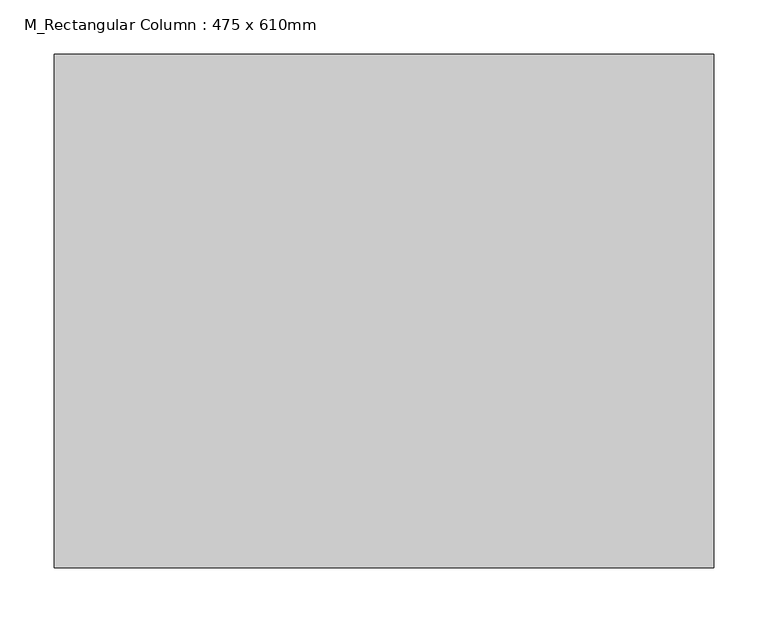
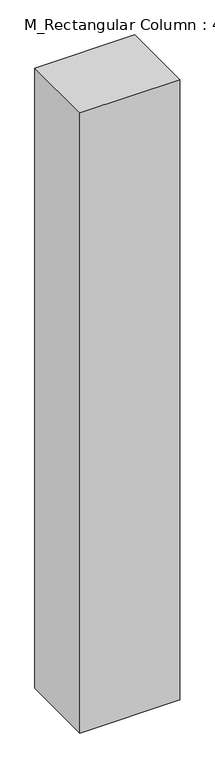
"""IFC4 building model written with IfcOpenShell, lengths in millimetres: column geometry, M_Rectangular Column : 475 x 610mm."""

import ifcopenshell
import ifcopenshell.guid

model = None  # the IFC model being written
_history = None  # IfcOwnerHistory: only IFC2X3 demands one
_inside = {}  # id of a spatial element -> (the spatial element, [elements in it])
_under = {}  # id of a project, library or spatial element -> (it, [spatial elements below it])
_declared = {}  # id of a project -> (the project, [libraries it declares])
_typed = {}  # id of a type object -> (the type object, [elements of that type])
_made_of = {}  # id of a material, layer set ... -> (it, [elements and type objects made of it])


def new_model(schema):
    """Start an empty IFC model of exactly this schema.

    Asked for "IFC4X3", IfcOpenShell would pick the latest addendum, in which some entities
    have other attributes; the version numbers below select the first issue.
    IFC2X3 requires an IfcOwnerHistory on every rooted entity: one is made here for all.
    """
    global model, _history
    if schema == "IFC4X3":
        model = ifcopenshell.file(schema_version=(4, 3, 0, 0))
    else:
        model = ifcopenshell.file(schema=schema)
    _inside.clear()
    _under.clear()
    _declared.clear()
    _typed.clear()
    _made_of.clear()
    _history = None
    if model.schema == "IFC2X3":
        org = make("IfcOrganization", Name="unknown")
        user = make(
            "IfcPersonAndOrganization",
            ThePerson=make("IfcPerson", FamilyName="unknown"),
            TheOrganization=org,
        )
        app = make(
            "IfcApplication",
            ApplicationDeveloper=org,
            Version="unknown",
            ApplicationFullName="unknown",
            ApplicationIdentifier="unknown",
        )
        _history = make(
            "IfcOwnerHistory",
            OwningUser=user,
            OwningApplication=app,
            ChangeAction="ADDED",
            CreationDate=0,
        )
    return model


def make(cls, **values):
    """One entity of the class cls with the attributes given. An attribute that is None is left unset."""
    return model.create_entity(
        cls, **{name: value for name, value in values.items() if value is not None}
    )


def rooted(cls, **values):
    """An entity with a GlobalId (a new one), such as an element, a storey or a relation."""
    return make(cls, GlobalId=ifcopenshell.guid.new(), OwnerHistory=_history, **values)


def si_unit(unit_type, name, prefix=None):
    """IfcSIUnit, for example si_unit("LENGTHUNIT", "METRE", prefix="MILLI")."""
    return make("IfcSIUnit", UnitType=unit_type, Prefix=prefix, Name=name)


def assignment(units):
    """IfcUnitAssignment: the units of a project."""
    return None if units is None else make("IfcUnitAssignment", Units=units)


def point(xyz):
    """IfcCartesianPoint."""
    return None if xyz is None else make("IfcCartesianPoint", Coordinates=xyz)


def direction(xyz):
    """IfcDirection."""
    return None if xyz is None else make("IfcDirection", DirectionRatios=xyz)


def frame(location, z_axis=None, x_axis=None):
    """IfcAxis2Placement3D, a coordinate frame: its origin and axes. An axis left out is left unset."""
    return make(
        "IfcAxis2Placement3D",
        Location=point(location),
        Axis=direction(z_axis),
        RefDirection=direction(x_axis),
    )


def origin():
    """The frame at (0, 0, 0) with its axes left unset."""
    return frame((0.0, 0.0, 0.0))


def place(relative_to, where):
    """IfcLocalPlacement: puts the frame where relative to a parent placement (None: the world)."""
    return make(
        "IfcLocalPlacement", PlacementRelTo=relative_to, RelativePlacement=where
    )


def context(
    kind, dimensions, precision=None, world=None, true_north=None, identifier=None
):
    """IfcGeometricRepresentationContext, for example the 3D "Model" context."""
    return make(
        "IfcGeometricRepresentationContext",
        ContextIdentifier=identifier,
        ContextType=kind,
        CoordinateSpaceDimension=dimensions,
        Precision=precision,
        WorldCoordinateSystem=world,
        TrueNorth=true_north,
    )


def project(units=None, contexts=None):
    """IfcProject with its units and contexts."""
    return rooted(
        "IfcProject",
        Name="project",
        RepresentationContexts=contexts,
        UnitsInContext=assignment(units),
    )


def spatial(cls, under=None, at=None, **own):
    """A site, building, storey or space (cls), placed at a placement, below another one or the project."""
    s = rooted(cls, ObjectPlacement=at, **own)
    if under is not None:
        _under.setdefault(under.id(), (under, []))[1].append(s)
    return s


def polyline(points):
    """IfcPolyline through the points."""
    return make("IfcPolyline", Points=[point(p) for p in points])


def outline(outer, holes=None, kind="AREA"):
    """IfcArbitraryClosedProfileDef: a profile drawn as a closed curve; with holes, ...WithVoids."""
    if holes is None:
        return make("IfcArbitraryClosedProfileDef", ProfileType=kind, OuterCurve=outer)
    return make(
        "IfcArbitraryProfileDefWithVoids",
        ProfileType=kind,
        OuterCurve=outer,
        InnerCurves=holes,
    )


def extrude(swept, where, along, depth):
    """IfcExtrudedAreaSolid: the profile swept, set in the frame where, extruded along a direction by depth."""
    return make(
        "IfcExtrudedAreaSolid",
        SweptArea=swept,
        Position=where,
        ExtrudedDirection=direction(along),
        Depth=depth,
    )


def shape(context_of_items, identifier, shape_type, items):
    """IfcShapeRepresentation: the items that make up one representation, for example the "Body"."""
    return make(
        "IfcShapeRepresentation",
        ContextOfItems=context_of_items,
        RepresentationIdentifier=identifier,
        RepresentationType=shape_type,
        Items=items,
    )


def source(mapping_origin, context_of_items, identifier, shape_type, items):
    """IfcRepresentationMap: a shape defined once, which mapped items show again and again."""
    return make(
        "IfcRepresentationMap",
        MappingOrigin=mapping_origin,
        MappedRepresentation=shape(context_of_items, identifier, shape_type, items),
    )


def transform(
    local_origin,
    x_axis=None,
    y_axis=None,
    z_axis=None,
    scale=None,
    scale2=None,
    scale3=None,
    uniform=True,
):
    """IfcCartesianTransformationOperator3D, or its non-uniform kind. x_axis, y_axis, z_axis: its Axis1, 2, 3."""
    if uniform:
        return make(
            "IfcCartesianTransformationOperator3D",
            Axis1=direction(x_axis),
            Axis2=direction(y_axis),
            LocalOrigin=point(local_origin),
            Scale=scale,
            Axis3=direction(z_axis),
        )
    return make(
        "IfcCartesianTransformationOperator3DnonUniform",
        Axis1=direction(x_axis),
        Axis2=direction(y_axis),
        LocalOrigin=point(local_origin),
        Scale=scale,
        Axis3=direction(z_axis),
        Scale2=scale2,
        Scale3=scale3,
    )


def mapped(mapping_source, mapping_target):
    """IfcMappedItem: shows the shape of a source again, moved by a transform."""
    return make(
        "IfcMappedItem", MappingSource=mapping_source, MappingTarget=mapping_target
    )


def made_of(thing, what):
    """Note that an element or type object is made of a material, layer set ...; save() writes the relation."""
    if what is not None:
        _made_of.setdefault(what.id(), (what, []))[1].append(thing)
    return thing


def element(
    cls,
    number,
    at=None,
    inside=None,
    cuts=None,
    type_object=None,
    material=None,
    context=None,
    identifier="Body",
    shape_type=None,
    held_by="IfcProductDefinitionShape",
    body=None,
    shapes=None,
    **own,
):
    """One element of the class cls, such as IfcWall. Its Tag is "e" and its number.

    at: its placement. inside: the storey or other place that contains it. cuts: it is an
    opening in that element (IfcRelVoidsElement). A single representation is given by context,
    identifier, shape_type and body (its items); several are given by shapes. held_by: the class
    of the entity that holds the representations. save() writes the other relations.
    """
    e = rooted(cls, Tag="e%d" % number, ObjectPlacement=at, **own)
    if body is not None:
        shapes = [shape(context, identifier, shape_type, body)]
    if shapes is not None:
        e.Representation = make(held_by, Representations=shapes)
    if inside is not None:
        _inside.setdefault(inside.id(), (inside, []))[1].append(e)
    if cuts is not None:
        rooted(
            "IfcRelVoidsElement", RelatingBuildingElement=cuts, RelatedOpeningElement=e
        )
    if type_object is not None:
        _typed.setdefault(type_object.id(), (type_object, []))[1].append(e)
    return made_of(e, material)


def aggregate(whole, parts):
    """IfcRelAggregates: a whole, such as a stair, and the parts it consists of."""
    return rooted("IfcRelAggregates", RelatingObject=whole, RelatedObjects=parts)


def save(model, path):
    """Write the relations noted so far, then the file.

    IfcRelAggregates (storeys below a building ...), IfcRelContainedInSpatialStructure (elements
    in a storey), IfcRelDefinesByType, IfcRelAssociatesMaterial and IfcRelDeclares: one each for
    every whole, place, type object, material and project.
    """
    for whole, parts in _under.values():
        aggregate(whole, parts)
    for where, things in _inside.values():
        rooted(
            "IfcRelContainedInSpatialStructure",
            RelatedElements=things,
            RelatingStructure=where,
        )
    for kind, things in _typed.values():
        rooted("IfcRelDefinesByType", RelatedObjects=things, RelatingType=kind)
    for what, things in _made_of.values():
        rooted("IfcRelAssociatesMaterial", RelatedObjects=things, RelatingMaterial=what)
    for by, libraries in _declared.values():
        rooted("IfcRelDeclares", RelatingContext=by, RelatedDefinitions=libraries)
    model.write(path)


def m_rectangular_column_475_x_610mm_e62a7db6(model_context):
    return source(origin(), model_context, "Body", "SweptSolid", [
        extrude(outline(polyline([(305.0, 237.5), (305.0, -237.5), (-305.0, -237.5), (-305.0, 237.5), (305.0, 237.5)])), frame((0.0, 0.0, 2000.0), z_axis=(0.0, 0.0, 1.0), x_axis=(1.0, 0.0, 0.0)), (0.0, 0.0, 1.0), 4000.0),
    ])


if __name__ == "__main__":
    model = new_model("IFC4")
    model_context = context("Model", 3, world=origin())
    ifc_project = project(units=[si_unit("LENGTHUNIT", "METRE", prefix="MILLI")], contexts=[model_context])
    site = spatial("IfcSite", under=ifc_project)
    building = spatial("IfcBuilding", under=site)
    placement = place(None, origin())
    m_rectangular_column_475_x_610mm_shape = m_rectangular_column_475_x_610mm_e62a7db6(model_context)
    element("IfcColumn", 1, ObjectType="M_Rectangular Column : 475 x 610mm", at=placement, inside=building, context=model_context, shape_type="MappedRepresentation", body=[
        mapped(m_rectangular_column_475_x_610mm_shape, transform((0.0, 0.0, 0.0), x_axis=(1.0, 0.0, 0.0), y_axis=(0.0, 1.0, 0.0), z_axis=(0.0, 0.0, 1.0))),
    ])
    save(model, "model.ifc")

# Revit data of these elements
# Type "M_Rectangular Column : 475 x 610mm"
#   Depth = 475 mm
#   Offset Base = 0 mm
#   Offset Top = 0 mm
#   Width = 610 mm
#   Material = none
